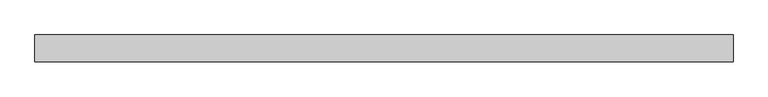
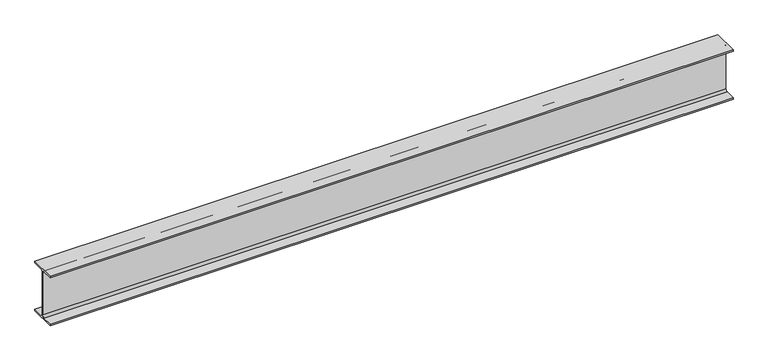
"""IFC4 building model written with IfcOpenShell, lengths in millimetres: beam geometry, 0912_Steel Framing_H-KSD3502 : H_SB_AR_S02_H-350x175x7x11_Platform."""

from ifc_helpers import new_model, si_unit, point, frame, frame_2d, origin, place, context, project, spatial, polyline, circle_curve, trimmed, segment, composite_curve, outline, extrude, source, transform, mapped, element, save


def beam_94df1702(model_context):
    return source(origin(), model_context, "Body", "SweptSolid", [
        extrude(outline(composite_curve([segment(polyline([(87.5, -164.0), (87.5, -175.0), (-87.5, -175.0), (-87.5, -164.0), (-17.5, -164.0)]), True, "CONTINUOUS"), segment(trimmed(circle_curve(frame_2d((-17.5, -150.0)), 14.0), [point((-17.5, -164.0))], [point((-3.5, -150.0))], True, "CARTESIAN"), True, "CONTINUOUS"), segment(polyline([(-3.5, -150.0), (-3.5, 150.0)]), True, "CONTINUOUS"), segment(trimmed(circle_curve(frame_2d((-17.5, 150.0)), 14.0), [point((-3.5, 150.0))], [point((-17.5, 164.0))], True, "CARTESIAN"), True, "CONTINUOUS"), segment(polyline([(-17.5, 164.0), (-87.5, 164.0), (-87.5, 175.0), (87.5, 175.0), (87.5, 164.0), (17.5, 164.0)]), True, "CONTINUOUS"), segment(trimmed(circle_curve(frame_2d((17.5, 150.0)), 14.0), [point((17.5, 164.0))], [point((3.5, 150.0))], True, "CARTESIAN"), True, "CONTINUOUS"), segment(polyline([(3.5, 150.0), (3.5, -150.0)]), True, "CONTINUOUS"), segment(trimmed(circle_curve(frame_2d((17.5, -150.0)), 14.0), [point((3.5, -150.0))], [point((17.5, -164.0))], True, "CARTESIAN"), True, "CONTINUOUS"), segment(polyline([(17.5, -164.0), (87.5, -164.0)]), True, "CONTINUOUS")], self_intersect=False)), frame((-2261.8008094, 0.0, 0.0), z_axis=(1.0, 0.0, 0.0), x_axis=(0.0, 1.0, 0.0)), (0.0, 0.0, 1.0), 4568.4611041),
    ])


if __name__ == "__main__":
    model = new_model("IFC4")
    model_context = context("Model", 3, world=origin())
    ifc_project = project(units=[si_unit("LENGTHUNIT", "METRE", prefix="MILLI")], contexts=[model_context])
    site = spatial("IfcSite", under=ifc_project)
    building = spatial("IfcBuilding", under=site)
    placement = place(None, origin())
    beam_shape = beam_94df1702(model_context)
    element("IfcBeam", 1, ObjectType="0912_Steel Framing_H-KSD3502 : H_SB_AR_S02_H-350x175x7x11_Platform", at=placement, inside=building, context=model_context, shape_type="MappedRepresentation", body=[
        mapped(beam_shape, transform((0.0, 0.0, 0.0), x_axis=(1.0, 0.0, 0.0), y_axis=(0.0, 1.0, 0.0), z_axis=(0.0, 0.0, 1.0))),
    ])
    save(model, "model.ifc")

# Revit data of these elements
# Type "0912_Steel Framing_H-KSD3502 : H_SB_AR_S02_H-350x175x7x11_Platform"
#   H_Q'ty Cal Type Tag = "SB-Q2"
#   H_WM Code_1 = "S01AA073-00001 |  | TON | Main Steel Structure Fabrication Work | Shelter/Building | Medium Steel - Standard |  |  |  |  |  |  | Material: (   ) | (90)KG/M>Weight≥(30)KG/M | S01AA073-00001 Main Steel Structure Fabrication Work Shelter/Building Medium Steel - Standard         | - Material: ( ASTM A36 )\n- (90)KG/M>Weight≥(30)KG/M"
#   H_WM Code_2 = "S03AA083-00001 |  | TON | Main Steel Structure Erection Work | Shelter/Building | Medium Steel |  |  |  |  |  |  | Material: (   ) | S03AA083-00001 Main Steel Structure Erection Work Shelter/Building Medium Steel         | - Material: ( ASTM A36 )"
#   H_WM Code_3 = "S01AA009-00001 |  | TON | Main Steel Structure Fabrication Work | Shelter/Building | Plates - Gusset, Stiffener, ETC | Material: (   ) | S01AA009-00001 Main Steel Structure Fabrication Work Shelter/Building Plates - Gusset, Stiffener, ETC         |"
#   H_WM Code_4 = "S41AA051-00001 |  | M2 | Steel Structure Paint Work | Shelter/Building | for Non-Fireproofed Steel Surface |  |  |  |  |  |  | Material: (   ) | S41AA051-00001 Steel Structure Paint Work Shelter/Building for Non-Fireproofed Steel Surface         |"
#   Width = 17.5 cm
#   Web Thickness = 0.7 cm
#   Web Fillet = 1.4 cm
#   Warping Constant = 282000.0 cm⁶
#   W = 0
#   Torsional Moment of Inertia = 19.4042 cm⁴
#   Section Area = 63.14 cm²
#   Plastic Modulus weak axis = 174.0 cm³
#   Plastic Modulus strong axis = 868.0 cm³
#   Perimeter = 1.36 m²/m
#   Nominal Weight = 49.60 kgf/m
#   Moment of Inertia weak axis = 984.00 cm⁴
#   Moment of Inertia strong axis = 13600.00 cm⁴
#   Height = 35.0 cm
#   Flange Thickness = 1.1 cm
#   Elastic Modulus weak axis = 112.0 cm³
#   Elastic Modulus strong axis = 775.0 cm³
#   Centroid Vertical = 17.5 cm
#   Centroid Horizontal = 8.75 cm
#   Ix = 136000000
#   Length [instance default] = 1524 mm
#   Zx = 868000
#   b = 175 mm
#   h = 350 mm
#   r = 14 mm
#   s = 7 mm
#   t = 11 mm
#   A = 0.006314 m²
#   Structural Material [instance default] = Steel, 45-345
#   Assembly Code = ""
# Element 1 (IfcBeam, "0912_Steel Framing_H-KSD3502 : H_SB_AR_S02_H-350x175x7x11_Platform")
#   Materials on its faces: "Steel, 45-345"
# Materials
#   "Steel, 45-345": class "Metal", colour RGB 189 187 185, transparency 0, Description = "Steel 345 MPa", Cost = 0
